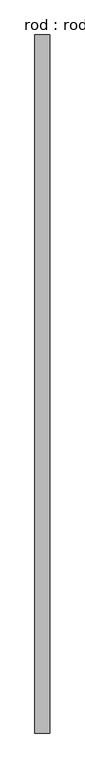
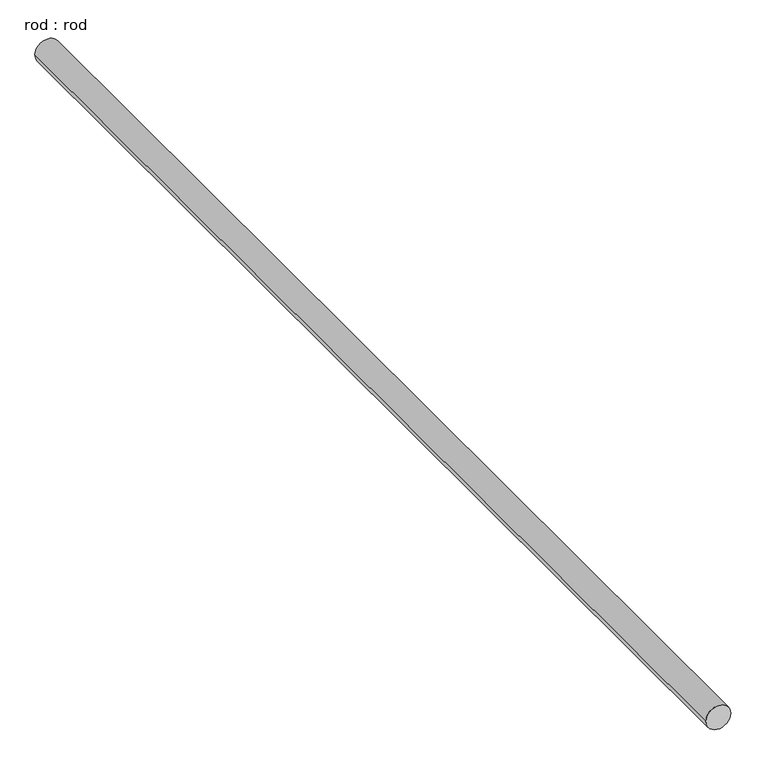
"""IFC4 building model written with IfcOpenShell, lengths in millimetres: proxy geometry, rod : rod."""

from ifc_helpers import new_model, si_unit, point, frame, frame_2d, origin, place, context, project, spatial, circle_curve, trimmed, segment, composite_curve, outline, extrude, source, transform, mapped, element, save


def rod_rod_acb5d2f3(model_context):
    return source(origin(), model_context, "Body", "SweptSolid", [
        extrude(outline(composite_curve([segment(trimmed(circle_curve(frame_2d((0.0108462, 0.0)), 200.0), [point((0.0108462, 200.0))], [point((0.0108462, -200.0))], False, "CARTESIAN"), True, "CONTINUOUS"), segment(trimmed(circle_curve(frame_2d((0.0108462, 0.0)), 200.0), [point((0.0108462, -200.0))], [point((0.0108462, 200.0))], False, "CARTESIAN"), True, "CONTINUOUS")], self_intersect=False)), frame((0.0, -5307.2713847, 0.0), z_axis=(0.0, 1.0, 0.0), x_axis=(0.0, 0.0, 1.0)), (0.0, 0.0, 1.0), 18800.0),
    ])


if __name__ == "__main__":
    model = new_model("IFC4")
    model_context = context("Model", 3, world=origin())
    ifc_project = project(units=[si_unit("LENGTHUNIT", "METRE", prefix="MILLI")], contexts=[model_context])
    site = spatial("IfcSite", under=ifc_project)
    building = spatial("IfcBuilding", under=site)
    placement = place(None, origin())
    rod_rod_shape = rod_rod_acb5d2f3(model_context)
    element("IfcBuildingElementProxy", 1, Name="rod : rod", ObjectType="rod : rod", at=placement, inside=building, context=model_context, shape_type="MappedRepresentation", body=[
        mapped(rod_rod_shape, transform((0.0, 0.0, 0.0), x_axis=(1.0, 0.0, 0.0), y_axis=(0.0, 1.0, 0.0), z_axis=(0.0, 0.0, 1.0))),
    ])
    save(model, "model.ifc")

# Revit data of these elements
# Type "rod : rod"
#   Default Elevation = 0
